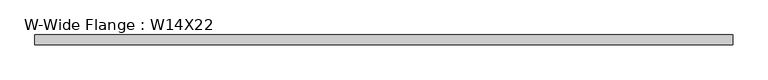
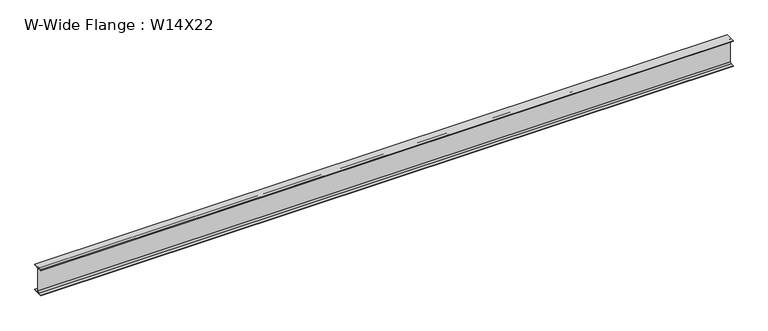
"""IFC4 building model written with IfcOpenShell, lengths in millimetres: beam geometry, W-Wide Flange : W14X22."""

from ifc_helpers import new_model, si_unit, point, frame, frame_2d, origin, place, context, project, spatial, polyline, circle_curve, trimmed, segment, composite_curve, outline, extrude, source, transform, mapped, element, save


def w_wide_flange_w14x22_2ac3afcd(model_context):
    return source(origin(), model_context, "Body", "SweptSolid", [
        extrude(outline(composite_curve([segment(polyline([(63.5, -165.481), (63.5, -173.99), (-63.5, -173.99), (-63.5, -165.481), (-21.3995, -165.481)]), True, "CONTINUOUS"), segment(trimmed(circle_curve(frame_2d((-21.3995, -147.0025)), 18.4785), [point((-21.3995, -165.481))], [point((-2.921, -147.0025))], True, "CARTESIAN"), True, "CONTINUOUS"), segment(polyline([(-2.921, -147.0025), (-2.921, 147.0025)]), True, "CONTINUOUS"), segment(trimmed(circle_curve(frame_2d((-21.3995, 147.0025)), 18.4785), [point((-2.921, 147.0025))], [point((-21.3995, 165.481))], True, "CARTESIAN"), True, "CONTINUOUS"), segment(polyline([(-21.3995, 165.481), (-63.5, 165.481), (-63.5, 173.99), (63.5, 173.99), (63.5, 165.481), (21.3995, 165.481)]), True, "CONTINUOUS"), segment(trimmed(circle_curve(frame_2d((21.3995, 147.0025)), 18.4785), [point((21.3995, 165.481))], [point((2.921, 147.0025))], True, "CARTESIAN"), True, "CONTINUOUS"), segment(polyline([(2.921, 147.0025), (2.921, -147.0025)]), True, "CONTINUOUS"), segment(trimmed(circle_curve(frame_2d((21.3995, -147.0025)), 18.4785), [point((2.921, -147.0025))], [point((21.3995, -165.481))], True, "CARTESIAN"), True, "CONTINUOUS"), segment(polyline([(21.3995, -165.481), (63.5, -165.481)]), True, "CONTINUOUS")], self_intersect=False)), frame((-4381.4503906, 0.0, 0.0), z_axis=(1.0, 0.0, 0.0), x_axis=(0.0, 1.0, 0.0)), (0.0, 0.0, 1.0), 8839.1007812),
    ])


if __name__ == "__main__":
    model = new_model("IFC4")
    model_context = context("Model", 3, world=origin())
    ifc_project = project(units=[si_unit("LENGTHUNIT", "METRE", prefix="MILLI")], contexts=[model_context])
    site = spatial("IfcSite", under=ifc_project)
    building = spatial("IfcBuilding", under=site)
    placement = place(None, origin())
    w_wide_flange_w14x22_shape = w_wide_flange_w14x22_2ac3afcd(model_context)
    element("IfcBeam", 1, ObjectType="W-Wide Flange : W14X22", at=placement, inside=building, context=model_context, shape_type="MappedRepresentation", body=[
        mapped(w_wide_flange_w14x22_shape, transform((0.0, 0.0, 0.0), x_axis=(1.0, 0.0, 0.0), y_axis=(0.0, 1.0, 0.0), z_axis=(0.0, 0.0, 1.0))),
    ])
    save(model, "model.ifc")

# Revit data of these elements
# Type "W-Wide Flange : W14X22"
#   Assembly Code = "B10"
#   W = 22
#   Length [instance default] = 1524 mm
#   bf = 127 mm
#   d = 347.98 mm
#   k = 26.988 mm
#   k2 = 18.479 mm
#   tf = 8.509 mm
#   tw = 5.842 mm
#   A = 0.00418709 m²
#   Structural Material [instance default] = Steel ASTM A992
# Element 1 (IfcBeam, "W-Wide Flange : W14X22")
#   Structural Material = Aluminum, Anodized Red
#   Materials on its faces: "Aluminum, Anodized Red"
# Materials
#   "Steel ASTM A992": class "Metal", colour RGB 128 0 0, transparency 0, Description = "Structural steel 50ksi", Cost = 0
#   "Aluminum, Anodized Red": class "Metal", colour RGB 120 120 120, transparency 0, Description = "Anodized aluminum, red", Cost = 0
